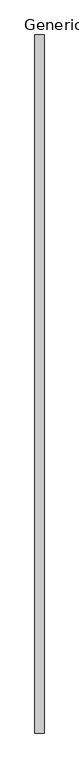
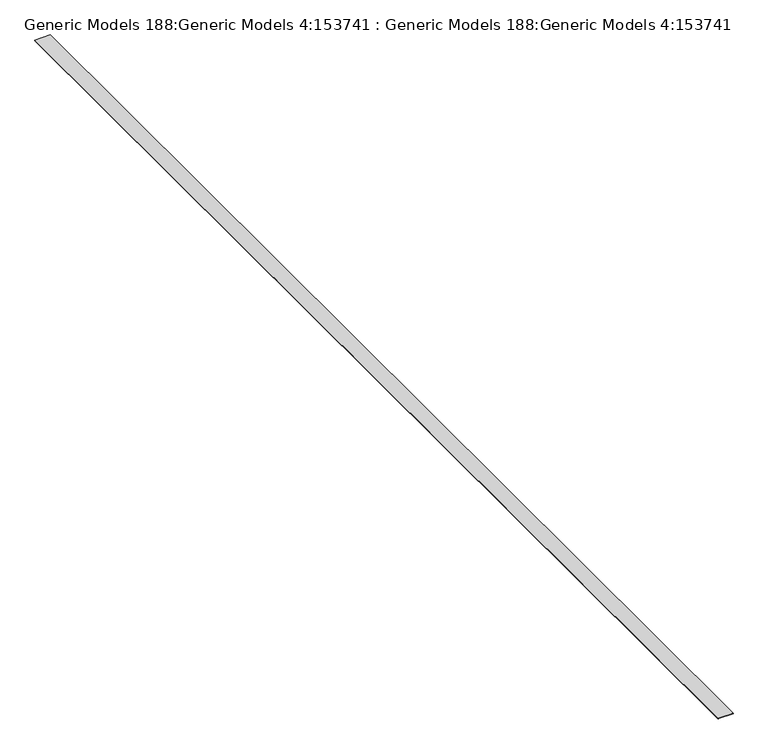
"""IFC4 building model written with IfcOpenShell, lengths in millimetres: proxy geometry, Generic Models 188:Generic Models 4:153741 : Generic Models 188:Generic Models 4:153741."""

from ifc_helpers import new_model, si_unit, frame, origin, place, context, project, spatial, polyline, outline, extrude, source, transform, mapped, element, save


def generic_models_188_generic_models_4_153741_generic_models_6dce9be7(model_context):
    return source(origin(), model_context, "Body", "SweptSolid", [
        extrude(outline(polyline([(-5246.3966051, 7612.7025207), (-5246.3966051, -273.9974793), (-5349.556089, -273.9974793), (-5349.556089, 7612.7025207), (-5246.3966051, 7612.7025207)])), frame((0.0, 0.0, 3474.1438466), z_axis=(0.0, 0.0, 1.0), x_axis=(1.0, 0.0, 0.0)), (0.0, 0.0, 1.0), 1.3753749),
        extrude(outline(polyline([(-5246.3966051, 7612.7025207), (-5246.3966051, -273.9974793), (-5349.556089, -273.9974793), (-5349.556089, 7612.7025207), (-5246.3966051, 7612.7025207)])), frame((0.0, 0.0, 3470.7501884), z_axis=(0.0, 0.0, 1.0), x_axis=(1.0, 0.0, 0.0)), (0.0, 0.0, 1.0), 1.3753749),
    ])


if __name__ == "__main__":
    model = new_model("IFC4")
    model_context = context("Model", 3, world=origin())
    ifc_project = project(units=[si_unit("LENGTHUNIT", "METRE", prefix="MILLI")], contexts=[model_context])
    site = spatial("IfcSite", under=ifc_project)
    building = spatial("IfcBuilding", under=site)
    placement = place(None, origin())
    generic_models_188_generic_models_4_153741_generic_models_shape = generic_models_188_generic_models_4_153741_generic_models_6dce9be7(model_context)
    element("IfcBuildingElementProxy", 1, Name="Generic Models 188:Generic Models 4:153741 : Generic Models 188:Generic Models 4:153741", ObjectType="Generic Models 188:Generic Models 4:153741 : Generic Models 188:Generic Models 4:153741", at=placement, inside=building, context=model_context, shape_type="MappedRepresentation", body=[
        mapped(generic_models_188_generic_models_4_153741_generic_models_shape, transform((0.0, 0.0, 0.0), x_axis=(1.0, 0.0, 0.0), y_axis=(0.0, 1.0, 0.0), z_axis=(0.0, 0.0, 1.0))),
    ])
    save(model, "model.ifc")

# Revit data of these elements
# Type "Generic Models 188:Generic Models 4:153741 : Generic Models 188:Generic Models 4:153741"
#   NameOverride = "Generic Models 188:Generic Models 4:153741"
#   ObjectTypeOverride = "Generic Models 188:Generic Models 4"
#   Reference = "Generic Models 4"
#   Category = "Generic Models"
#   Tag = "153741"
# Element 1 (IfcBuildingElementProxy, "Generic Models 188:Generic Models 4:153741 : Generic Models 188:Generic Models 4:153741")
#   Materials on its faces: "_BED OF SEALANT (ABOVE/BELOW FLASHING) 12592"
# Materials
#   "_BED OF SEALANT (ABOVE/BELOW FLASHING) 12592": class "Unassigned", colour RGB 253 192 103, transparency 0
